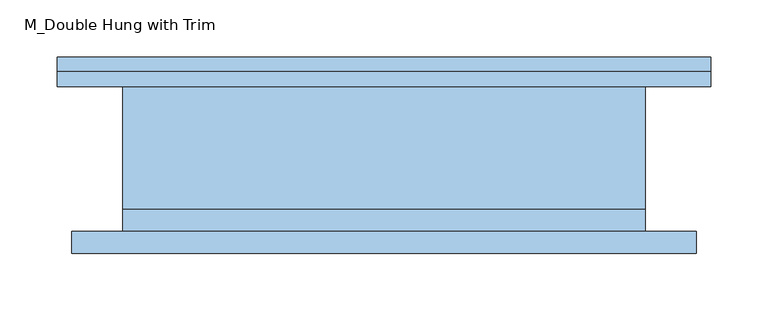
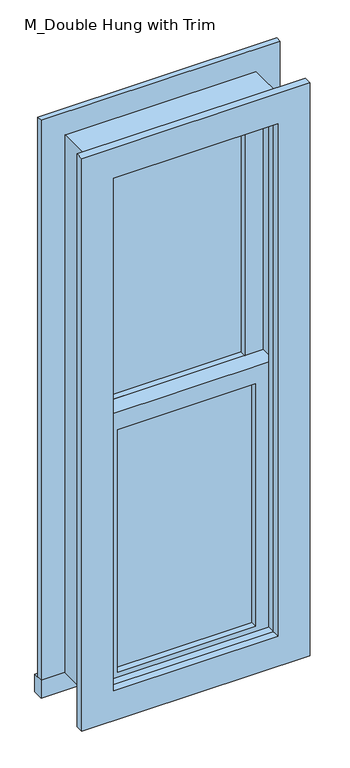
"""IFC4 building model written with IfcOpenShell, lengths in millimetres: window geometry, M_Double Hung with Trim."""

from ifc_helpers import new_model, si_unit, frame, origin, place, context, project, spatial, polyline, outline, extrude, source, transform, mapped, element, save


def m_double_hung_with_trim_7e06b87c(model_context):
    return source(origin(), model_context, "Body", "SweptSolid", [
        extrude(outline(polyline([(-165.1, -15.825), (165.1, -15.825), (165.1, -28.525), (-165.1, -28.525), (-165.1, -15.825)])), frame((0.0, 0.0, 628.65), z_axis=(0.0, 0.0, 1.0), x_axis=(1.0, 0.0, 0.0)), (0.0, 0.0, 1.0), 612.775),
        extrude(outline(polyline([(1285.875, -209.55), (584.2, -209.55), (584.2, 209.55), (1285.875, 209.55), (1285.875, -209.55)]), holes=[polyline([(1241.425, -165.1), (1241.425, 165.1), (628.65, 165.1), (628.65, -165.1), (1241.425, -165.1)])]), frame((0.0, -44.4, 0.0), z_axis=(0.0, 1.0, 0.0), x_axis=(0.0, 0.0, 1.0)), (0.0, 0.0, 1.0), 44.45),
        extrude(outline(polyline([(-285.75, 89.2), (285.75, 89.2), (285.75, 63.5), (-285.75, 63.5), (-285.75, 89.2)])), frame((0.0, 0.0, 539.75), z_axis=(0.0, 0.0, 1.0), x_axis=(1.0, 0.0, 0.0)), (0.0, 0.0, 1.0), 44.45),
        extrude(outline(polyline([(2000.25, -285.75), (539.75, -285.75), (539.75, 285.75), (2000.25, 285.75), (2000.25, -285.75)]), holes=[polyline([(1924.05, -209.55), (1924.05, 209.55), (584.2, 209.55), (584.2, -209.55), (1924.05, -209.55)])]), frame((0.0, 63.5, 0.0), z_axis=(0.0, 1.0, 0.0), x_axis=(0.0, 0.0, 1.0)), (0.0, 0.0, 1.0), 13.0),
        extrude(outline(polyline([(1987.55, 273.05), (1987.55, -273.05), (539.75, -273.05), (539.75, 273.05), (1987.55, 273.05)]), holes=[polyline([(1911.35, 196.85), (615.95, 196.85), (615.95, -196.85), (1911.35, -196.85), (1911.35, 196.85)])]), frame((0.0, -82.5, 0.0), z_axis=(0.0, 1.0, 0.0), x_axis=(0.0, 0.0, 1.0)), (0.0, 0.0, 1.0), 19.0),
        extrude(outline(polyline([(165.1, 15.925), (-165.1, 15.925), (-165.1, 28.625), (165.1, 28.625), (165.1, 15.925)])), frame((0.0, 0.0, 1285.875), z_axis=(0.0, 0.0, 1.0), x_axis=(1.0, 0.0, 0.0)), (0.0, 0.0, 1.0), 593.725),
        extrude(outline(polyline([(1924.05, -209.55), (1241.425, -209.55), (1241.425, 209.55), (1924.05, 209.55), (1924.05, -209.55)]), holes=[polyline([(1879.6, -165.1), (1879.6, 165.1), (1285.875, 165.1), (1285.875, -165.1), (1879.6, -165.1)])]), frame((0.0, 0.05, 0.0), z_axis=(0.0, 1.0, 0.0), x_axis=(0.0, 0.0, 1.0)), (0.0, 0.0, 1.0), 44.45),
        extrude(outline(polyline([(1943.1, -228.6), (584.2, -228.6), (584.2, 228.6), (1943.1, 228.6), (1943.1, -228.6)]), holes=[polyline([(1911.35, -196.85), (1911.35, 196.85), (615.95, 196.85), (615.95, -196.85), (1911.35, -196.85)])]), frame((0.0, -63.5, 0.0), z_axis=(0.0, 1.0, 0.0), x_axis=(0.0, 0.0, 1.0)), (0.0, 0.0, 1.0), 19.1),
        extrude(outline(polyline([(1943.1, 228.6), (1943.1, -228.6), (584.2, -228.6), (584.2, 228.6), (1943.1, 228.6)]), holes=[polyline([(1924.05, 209.55), (603.25, 209.55), (603.25, -209.55), (1924.05, -209.55), (1924.05, 209.55)])]), frame((0.0, -44.4, 0.0), z_axis=(0.0, 1.0, 0.0), x_axis=(0.0, 0.0, 1.0)), (0.0, 0.0, 1.0), 107.9),
    ])


if __name__ == "__main__":
    model = new_model("IFC4")
    model_context = context("Model", 3, world=origin())
    ifc_project = project(units=[si_unit("LENGTHUNIT", "METRE", prefix="MILLI")], contexts=[model_context])
    site = spatial("IfcSite", under=ifc_project)
    building = spatial("IfcBuilding", under=site)
    placement = place(None, origin())
    m_double_hung_with_trim_shape = m_double_hung_with_trim_7e06b87c(model_context)
    element("IfcWindow", 1, ObjectType="M_Double Hung with Trim : 1'  6\" x 4'  5 1/2\"", at=placement, inside=building, context=model_context, shape_type="MappedRepresentation", body=[
        mapped(m_double_hung_with_trim_shape, transform((0.0, 0.0, 0.0), x_axis=(1.0, 0.0, 0.0), y_axis=(0.0, 1.0, 0.0), z_axis=(0.0, 0.0, 1.0))),
    ])
    save(model, "model.ifc")

# Revit data of these elements
# Type "M_Double Hung with Trim : 1'  6\" x 4'  5 1/2\""
#   Type Mark = "74"
#   Construction Type Id = "GSP4R"
#   Analytic Construction = "1/8 in Pilkington single glazing"
#   Visual Light Transmittance = 0.9
#   Thermal Resistance (R) = 0.271106 (m²·K)/W
#   Solar Heat Gain Coefficient = 0.78
#   Heat Transfer Coefficient (U) = 3.6886 W/(m²·K)
#   Height = 4' - 5 1/2"
#   Default Sill Height = 1' - 11"
#   Trim Projection - Ext. = 0' - 0.51181"
#   Trim Projection - Int. = 0' - 0.74803"
#   Trim Width - Exterior = 0' - 3"
#   Trim Width - Interior = 0' - 3"
#   Width = 1' - 6"
#   Window Inset = 0' - 0.74803"
#   Glass Pane Material = EXISTING WINDOW
#   Sash = Trim
#   Trim Exterior Material = Trim
#   Trim Interior Material = Trim
#   Wall Closure = (empty or 0)
# Element 1 (IfcWindow, "M_Double Hung with Trim : 1'  6\" x 4'  5 1/2\"")
#   Materials on its faces: "Trim", "EXISTING WINDOW"
# Materials
#   "EXISTING WINDOW": class "Glass", colour RGB 218 227 224, transparency 0.85, Description = "Soda Lime Glass", Cost = 0
#   "Trim": class "Wood", colour RGB 250 251 245, transparency 0, Cost = 0
